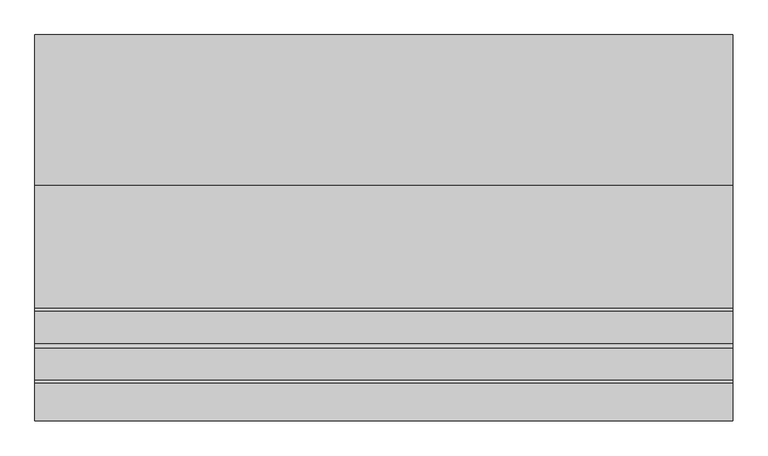
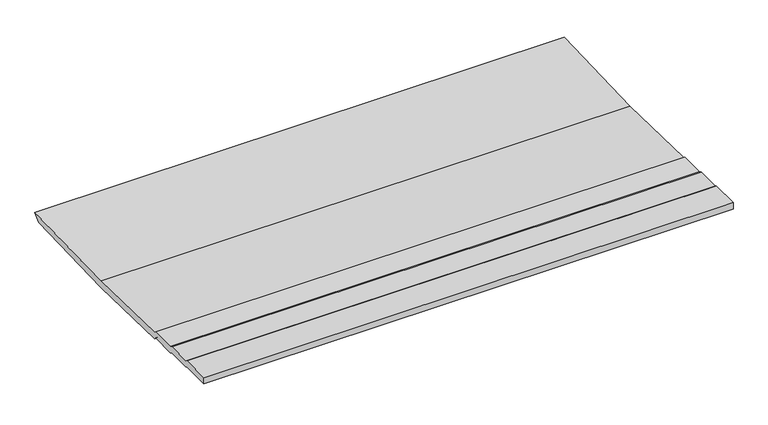
"""IFC4 building model written with IfcOpenShell, lengths in millimetres: proxy geometry, GRAVEL BALLAST002 34887 : GRAVEL BALLAST002 34887."""

from ifc_helpers import new_model, si_unit, frame, origin, place, context, project, spatial, polyline, outline, extrude, source, transform, mapped, element, save


def generic_models_c19f6b3d(model_context):
    return source(origin(), model_context, "Body", "SweptSolid", [
        extrude(outline(polyline([(-5440.365918, 40253.79375), (-5549.8654297, 40253.79375), (-5549.8654297, 40278.5320313), (-5440.365918, 40278.5320313), (-5431.6554687, 40274.2507813), (-5341.0685547, 40274.2507813), (-5328.2239153, 40268.5233193), (-5234.272168, 40270.16875), (-5225.9987305, 40262.7585938), (-4873.4420898, 40254.5398438), (-4442.8393555, 40268.1982422), (-4468.0649414, 40242.9726562), (-4873.4420898, 40229.8015625), (-5225.9987305, 40238.0203125), (-5234.272168, 40245.4304687), (-5328.2239153, 40243.785038), (-5341.0685547, 40249.5125), (-5431.6554687, 40249.5125), (-5440.365918, 40253.79375)])), frame((12382.7678845, 0.0, 0.0), z_axis=(1.0, 0.0, 0.0), x_axis=(0.0, 1.0, 0.0)), (0.0, 0.0, 1.0), 2000.0),
    ])


if __name__ == "__main__":
    model = new_model("IFC4")
    model_context = context("Model", 3, world=origin())
    ifc_project = project(units=[si_unit("LENGTHUNIT", "METRE", prefix="MILLI")], contexts=[model_context])
    site = spatial("IfcSite", under=ifc_project)
    building = spatial("IfcBuilding", under=site)
    placement = place(None, origin())
    generic_models_shape = generic_models_c19f6b3d(model_context)
    element("IfcBuildingElementProxy", 1, Name="GRAVEL BALLAST002 34887 : GRAVEL BALLAST002 34887", ObjectType="GRAVEL BALLAST002 34887 : GRAVEL BALLAST002 34887", at=placement, inside=building, context=model_context, shape_type="MappedRepresentation", body=[
        mapped(generic_models_shape, transform((0.0, 0.0, 0.0), x_axis=(1.0, 0.0, 0.0), y_axis=(0.0, 1.0, 0.0), z_axis=(0.0, 0.0, 1.0))),
    ])
    save(model, "model.ifc")

# Revit data of these elements
# Type "GRAVEL BALLAST002 34887 : GRAVEL BALLAST002 34887"
#   NameOverride = "GRAVEL BALLAST002"
# Element 1 (IfcBuildingElementProxy, "GRAVEL BALLAST002 34887 : GRAVEL BALLAST002 34887")
#   Materials on its faces: "GRAVEL BALLAST"
# Materials
#   "GRAVEL BALLAST": class "Unassigned", colour RGB 128 128 128, transparency 0, Cost = 0
